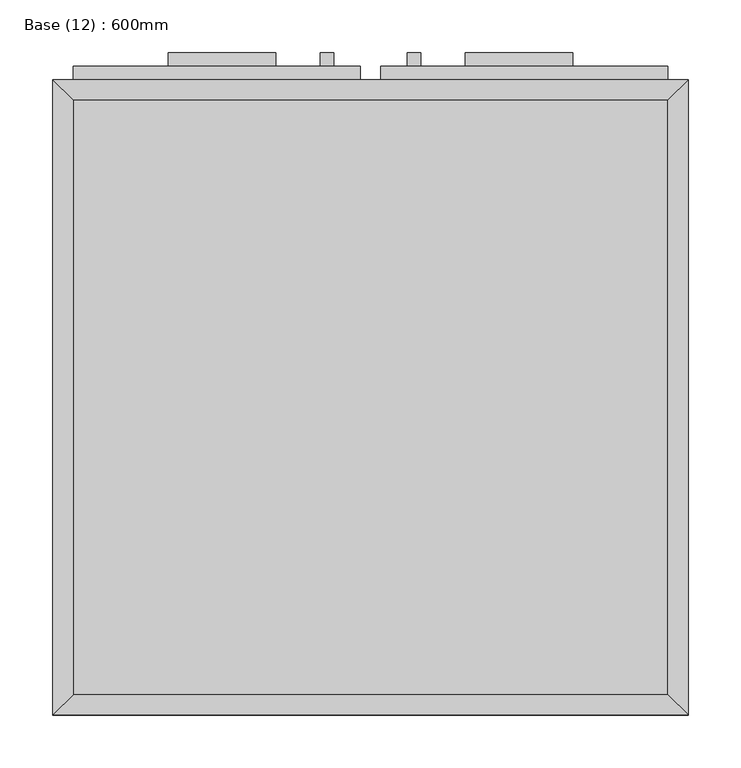
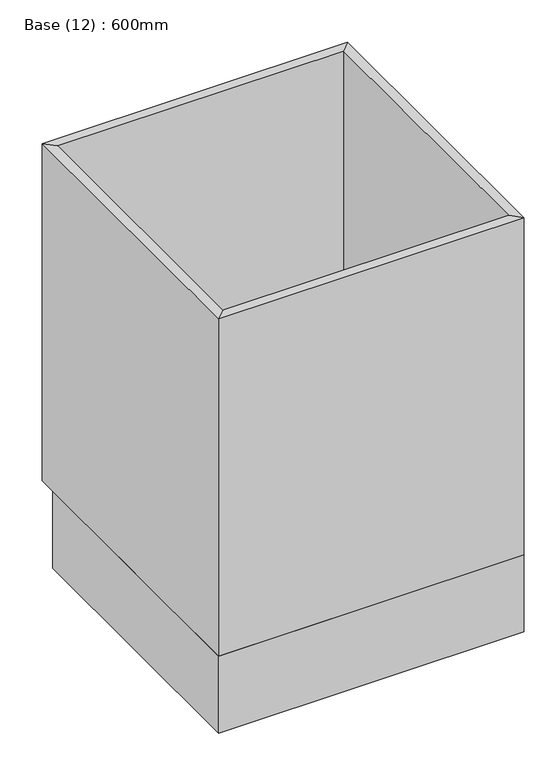
"""IFC4 building model written with IfcOpenShell, lengths in millimetres: furniture geometry, Base (12) : 600mm."""

from ifc_helpers import new_model, si_unit, frame, origin, origin_with_axes, place, context, project, spatial, polyline, outline, extrude, faceted_brep, source, transform, mapped, element, save


def base_12_600mm_73813d14(model_context):
    return source(origin(), model_context, "Body", "SolidModel", [
        extrude(outline(polyline([(299.6877049, 19.05), (-262.2122951, 19.05), (-262.2122951, 580.95), (299.6877049, 580.95), (299.6877049, 19.05)])), frame((0.0, 0.0, 160.0), z_axis=(0.0, 0.0, 1.0), x_axis=(1.0, 0.0, 0.0)), (0.0, 0.0, 1.0), 19.05),
        faceted_brep([(299.6877049, 580.95, 860.0), (-262.2122951, 580.95, 860.0), (-262.2122951, 580.95, 160.0), (299.6877049, 580.95, 160.0), (318.7377049, 600.0, 860.0), (-281.2622951, 600.0, 860.0), (318.7377049, 600.0, 160.0), (-281.2622951, 600.0, 160.0), (-262.2122951, 19.05, 860.0), (-262.2122951, 19.05, 160.0), (-281.2622951, 0.0, 860.0), (-281.2622951, 0.0, 160.0), (299.6877049, 19.05, 860.0), (299.6877049, 19.05, 160.0), (318.7377049, 0.0, 860.0), (318.7377049, 0.0, 160.0)], [[[0, 1, 2, 3]], [[4, 5, 1, 0]], [[6, 7, 5, 4]], [[3, 2, 7, 6]], [[1, 8, 9, 2]], [[5, 10, 8, 1]], [[7, 11, 10, 5]], [[2, 9, 11, 7]], [[8, 12, 13, 9]], [[10, 14, 12, 8]], [[11, 15, 14, 10]], [[9, 13, 15, 11]], [[12, 0, 3, 13]], [[14, 4, 0, 12]], [[15, 6, 4, 14]], [[13, 3, 6, 15]]]),
        extrude(outline(polyline([(318.7377049, 0.0), (-281.2622951, 0.0), (-281.2622951, 565.0), (318.7377049, 565.0), (318.7377049, 0.0)])), origin_with_axes(), (0.0, 0.0, 1.0), 160.0),
        extrude(outline(polyline([(-70.9372951, 625.4), (-70.9372951, 612.7), (-172.5372951, 612.7), (-172.5372951, 625.4), (-70.9372951, 625.4)])), frame((0.0, 0.0, 802.85), z_axis=(0.0, 0.0, 1.0), x_axis=(1.0, 0.0, 0.0)), (0.0, 0.0, 1.0), 12.7),
        extrude(outline(polyline([(210.0127049, 625.4), (210.0127049, 612.7), (108.4127049, 612.7), (108.4127049, 625.4), (210.0127049, 625.4)])), frame((0.0, 0.0, 802.85), z_axis=(0.0, 0.0, 1.0), x_axis=(1.0, 0.0, 0.0)), (0.0, 0.0, 1.0), 12.7),
        extrude(outline(polyline([(-16.1872951, 625.4), (-16.1872951, 612.7), (-28.8872951, 612.7), (-28.8872951, 625.4), (-16.1872951, 625.4)])), frame((0.0, 0.0, 580.6), z_axis=(0.0, 0.0, 1.0), x_axis=(1.0, 0.0, 0.0)), (0.0, 0.0, 1.0), 101.6),
        extrude(outline(polyline([(66.3627049, 625.4), (66.3627049, 612.7), (53.6627049, 612.7), (53.6627049, 625.4), (66.3627049, 625.4)])), frame((0.0, 0.0, 580.6), z_axis=(0.0, 0.0, 1.0), x_axis=(1.0, 0.0, 0.0)), (0.0, 0.0, 1.0), 101.6),
        extrude(outline(polyline([(9.2127049, 612.7), (9.2127049, 600.0), (-262.2122951, 600.0), (-262.2122951, 612.7), (9.2127049, 612.7)])), frame((0.0, 0.0, 739.35), z_axis=(0.0, 0.0, 1.0), x_axis=(1.0, 0.0, 0.0)), (0.0, 0.0, 1.0), 101.6),
        extrude(outline(polyline([(299.6877049, 612.7), (299.6877049, 600.0), (28.2627049, 600.0), (28.2627049, 612.7), (299.6877049, 612.7)])), frame((0.0, 0.0, 739.35), z_axis=(0.0, 0.0, 1.0), x_axis=(1.0, 0.0, 0.0)), (0.0, 0.0, 1.0), 101.6),
        extrude(outline(polyline([(9.2127049, 612.7), (9.2127049, 600.0), (-262.2122951, 600.0), (-262.2122951, 612.7), (9.2127049, 612.7)])), frame((0.0, 0.0, 179.05), z_axis=(0.0, 0.0, 1.0), x_axis=(1.0, 0.0, 0.0)), (0.0, 0.0, 1.0), 541.25),
        extrude(outline(polyline([(299.6877049, 612.7), (299.6877049, 600.0), (28.2627049, 600.0), (28.2627049, 612.7), (299.6877049, 612.7)])), frame((0.0, 0.0, 179.05), z_axis=(0.0, 0.0, 1.0), x_axis=(1.0, 0.0, 0.0)), (0.0, 0.0, 1.0), 541.25),
    ])


if __name__ == "__main__":
    model = new_model("IFC4")
    model_context = context("Model", 3, world=origin())
    ifc_project = project(units=[si_unit("LENGTHUNIT", "METRE", prefix="MILLI")], contexts=[model_context])
    site = spatial("IfcSite", under=ifc_project)
    building = spatial("IfcBuilding", under=site)
    placement = place(None, origin())
    base_12_600mm_shape = base_12_600mm_73813d14(model_context)
    element("IfcFurniture", 1, ObjectType="Base (12) : 600mm", at=placement, inside=building, context=model_context, shape_type="MappedRepresentation", body=[
        mapped(base_12_600mm_shape, transform((0.0, 0.0, 0.0), x_axis=(1.0, 0.0, 0.0), y_axis=(0.0, 1.0, 0.0), z_axis=(0.0, 0.0, 1.0))),
    ])
    save(model, "model.ifc")

# Revit data of these elements
# Type "Base (12) : 600mm"
#   Keynote = "N10"
#   Depth = 600 mm
#   Height = 860 mm
#   Plinth Depth = 35 mm
#   Plinth Height = 160 mm
#   Width = 600 mm
#   Material Cabinet = Cabinets
#   Material Door/Drawer = Cabinets
#   Material Handle = Cabinets - Handles
# Element 1 (IfcFurniture, "Base (12) : 600mm")
#   Materials on its faces: "Cabinets", "Cabinets - Handles"
# Materials
#   "Cabinets": class "Miscellaneous", colour RGB 249 249 249, transparency 0
#   "Cabinets - Handles": class "Metal", colour RGB 57 57 57, transparency 0
